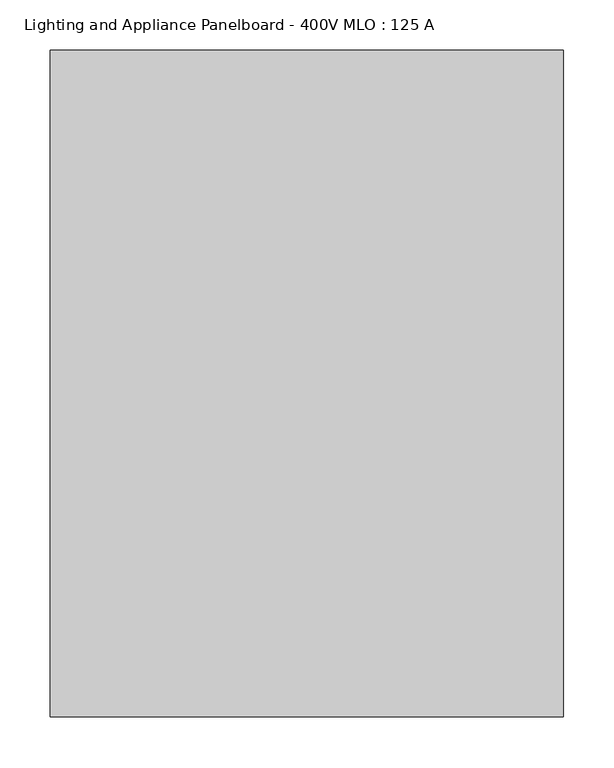
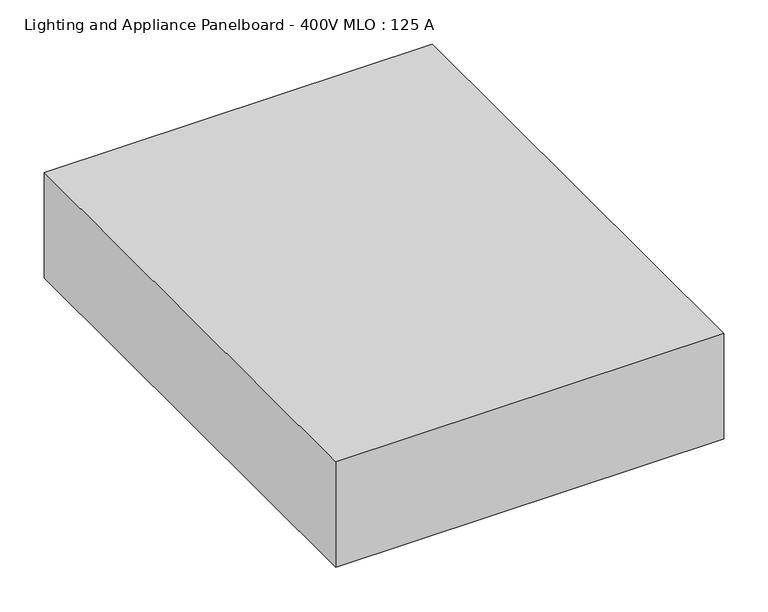
"""IFC4 building model written with IfcOpenShell, lengths in millimetres: proxy geometry, Lighting and Appliance Panelboard - 400V MLO : 125 A."""

from ifc_helpers import new_model, si_unit, frame, origin, place, context, project, spatial, polyline, outline, extrude, source, transform, mapped, element, save


def lighting_and_appliance_panelboard_400v_mlo_125_a_11cb7106(model_context):
    return source(origin(), model_context, "Body", "SweptSolid", [
        extrude(outline(polyline([(254.0, -660.4), (-254.0, -660.4), (-254.0, 0.0), (254.0, 0.0), (254.0, -660.4)])), frame((0.0, 0.0, -146.1), z_axis=(0.0, 0.0, 1.0), x_axis=(1.0, 0.0, 0.0)), (0.0, 0.0, 1.0), 146.1),
    ])


if __name__ == "__main__":
    model = new_model("IFC4")
    model_context = context("Model", 3, world=origin())
    ifc_project = project(units=[si_unit("LENGTHUNIT", "METRE", prefix="MILLI")], contexts=[model_context])
    site = spatial("IfcSite", under=ifc_project)
    building = spatial("IfcBuilding", under=site)
    placement = place(None, origin())
    lighting_and_appliance_panelboard_400v_mlo_125_a_shape = lighting_and_appliance_panelboard_400v_mlo_125_a_11cb7106(model_context)
    element("IfcBuildingElementProxy", 1, Name="Lighting and Appliance Panelboard - 400V MLO : 125 A", ObjectType="Lighting and Appliance Panelboard - 400V MLO : 125 A", at=placement, inside=building, context=model_context, shape_type="MappedRepresentation", body=[
        mapped(lighting_and_appliance_panelboard_400v_mlo_125_a_shape, transform((0.0, 0.0, 0.0), x_axis=(1.0, 0.0, 0.0), y_axis=(0.0, 1.0, 0.0), z_axis=(0.0, 0.0, 1.0))),
    ])
    save(model, "model.ifc")

# Revit data of these elements
# Type "Lighting and Appliance Panelboard - 400V MLO : 125 A"
#   built-in parameter 1140081 [instance default] = "Recessed"
#   built-in parameter 1140083 [instance default] = "Type 1"
#   Width = 508 mm
#   built-in parameter 1140082 [instance default] = 100 (stored number, unit not read)
#   built-in parameter 1140140 [instance default] = 1 (stored number, unit not read)
#   Height [instance default] = 660.4 mm
#   Depth = 146.1 mm
#   Default Elevation = 1200 mm
#   42 Circuit Height = 1117.6 mm
#   30 Circuit Height = 965.2 mm
#   18 Circuit Height = 660.4 mm
#   12 Circuit Height = 660.4 mm
#   built-in parameter 1140142 [instance default] = -1
#   built-in parameter 1140079 [instance default] = 12
#   built-in parameter 1155100 [instance default] = -1
#   Load Classification = Other
#   built-in parameter 1140087 [instance default] = element -7000014
